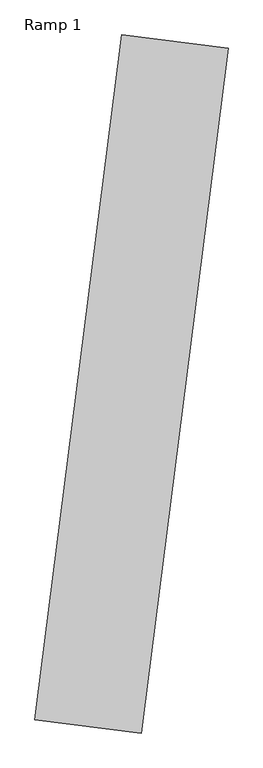
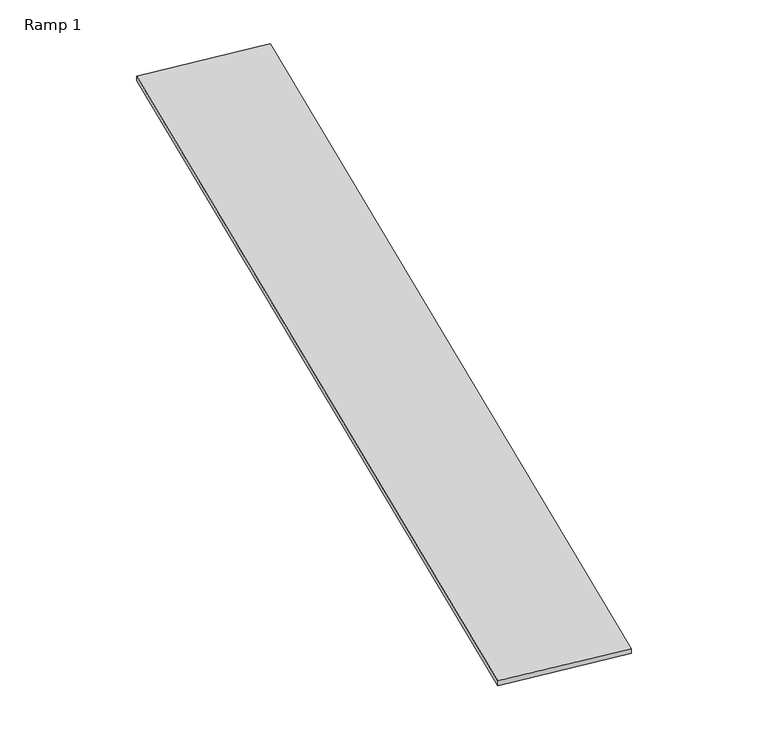
"""IFC4 building model written with IfcOpenShell, lengths in millimetres: ramp geometry, Ramp 1."""

from ifc_helpers import new_model, si_unit, frame, origin, place, context, project, spatial, polyline, outline, extrude, source, transform, mapped, element, save


def ramp_1_3ccef93f(model_context):
    return source(origin(), model_context, "Body", "SweptSolid", [
        extrude(outline(polyline([(-4700.0, -32182.9414905), (0.0, 0.0), (202.121519, 0.0), (-4497.878481, -32182.9414905), (-4700.0, -32182.9414905)])), frame((18351.118119, 124883.6460283, 5300.0), z_axis=(-0.9920606394423034, 0.12576043761584285, 0.0), x_axis=(0.0, 0.0, -1.0)), (0.0, 0.0, 1.0), 5000.0),
    ])


if __name__ == "__main__":
    model = new_model("IFC4")
    model_context = context("Model", 3, world=origin())
    ifc_project = project(units=[si_unit("LENGTHUNIT", "METRE", prefix="MILLI")], contexts=[model_context])
    site = spatial("IfcSite", under=ifc_project)
    building = spatial("IfcBuilding", under=site)
    placement = place(None, origin())
    ramp_1_shape = ramp_1_3ccef93f(model_context)
    element("IfcRamp", 1, ObjectType="Ramp 1", at=placement, inside=building, context=model_context, shape_type="MappedRepresentation", body=[
        mapped(ramp_1_shape, transform((0.0, 0.0, 0.0), x_axis=(1.0, 0.0, 0.0), y_axis=(0.0, 1.0, 0.0), z_axis=(0.0, 0.0, 1.0))),
    ])
    save(model, "model.ifc")
